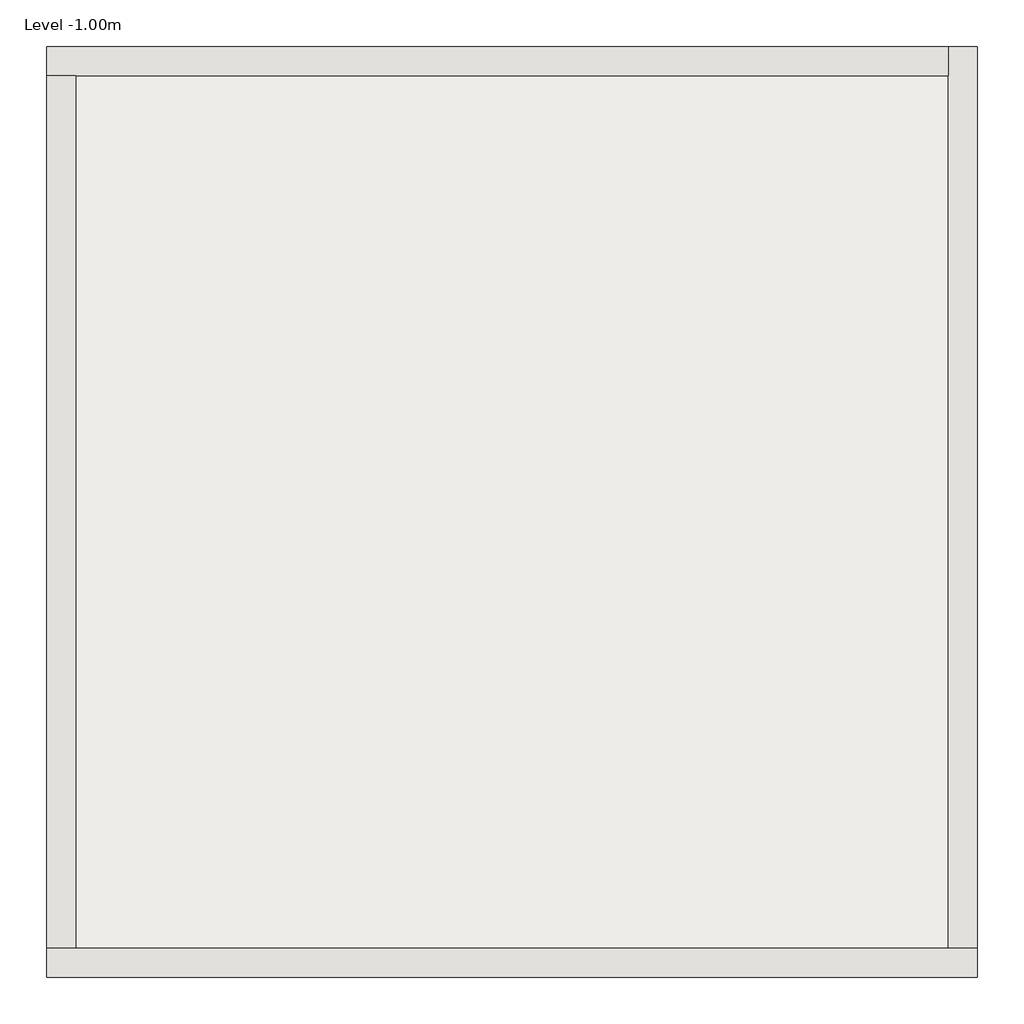
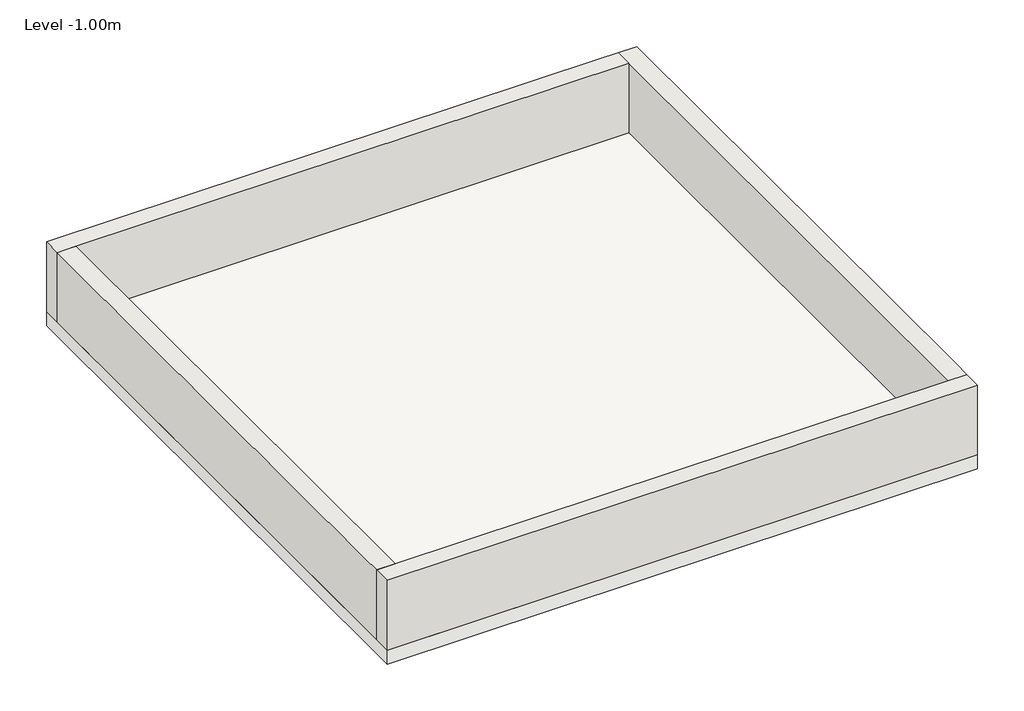
# One storey: 4 walls, 1 slab.
"""IFC4 building model written with IfcOpenShell, lengths in millimetres."""

from ifc_helpers import new_model, si_unit, frame, origin, place, context, project, spatial, polyline, outline, extrude, faceted_brep, element, save

model = new_model("IFC4")

# Units and contexts
model_context = context("Model", 3, world=origin())
ifc_project = project(units=[si_unit("LENGTHUNIT", "METRE", prefix="MILLI")], contexts=[model_context])

# Site, building, storey
site = spatial("IfcSite", under=ifc_project)
building = spatial("IfcBuilding", under=site)
storey = spatial("IfcBuildingStorey", under=building, Name="Level -1.00m", Elevation=-1000.0)

# Slab
placement = place(None, origin())
element("IfcSlab", 1, ObjectType="SOL CAM SANIT", at=placement, inside=storey, context=model_context, shape_type="SweptSolid", body=[
    extrude(outline(polyline([(0.0, 7999.99416), (7999.99416, 7999.99416), (7999.99416, 0.0), (0.0, 0.0), (0.0, 7999.99416)])), frame((0.0, 0.0, -1202.9999956), z_axis=(0.0, 0.0, 1.0), x_axis=(1.0, 0.0, 0.0)), (0.0, 0.0, 1.0), 202.9999956),
])

# Walls
element("IfcWall", 2, ObjectType="MURO CAM SANIT", at=placement, inside=storey, context=model_context, shape_type="Brep", body=[
    faceted_brep([(0.0, 0.0, -1000.0), (7999.99416, 0.0, -1000.0), (7999.99416, 0.0, -0.01216), (0.0, 0.0, -0.01216), (0.0, 249.000008, -1000.0), (0.0, 249.000008, -0.01216), (249.000008, 249.000008, -0.01216), (7750.994152, 249.000008, -0.01216), (7999.99416, 249.000008, -0.01216), (7999.99416, 249.000008, -1000.0), (7750.994152, 249.000008, -1000.0), (249.000008, 249.000008, -1000.0)], [[[0, 1, 2, 3]], [[4, 5, 6, 7, 8, 9, 10, 11]], [[1, 0, 4, 11, 10, 9]], [[3, 2, 8, 7, 6, 5]], [[2, 1, 9, 8]], [[0, 3, 5, 4]]]),
])
element("IfcWall", 3, ObjectType="MURO CAM SANIT", at=placement, inside=storey, context=model_context, shape_type="Brep", body=[
    faceted_brep([(7999.99416, 249.000008, -1000.0), (7999.99416, 7999.99416, -1000.0), (7999.99416, 7999.99416, -0.01216), (7999.99416, 500.000016, -0.01216), (7999.99416, 249.000008, -0.01216), (7750.994152, 249.000008, -1000.0), (7750.994152, 249.000008, -0.01216), (7750.994152, 7750.994152, -0.01216), (7750.994152, 7999.99416, -0.01216), (7750.994152, 7999.99416, -1000.0), (7750.994152, 7750.994152, -1000.0)], [[[0, 1, 2, 3, 4]], [[5, 6, 7, 8, 9, 10]], [[1, 0, 5, 10, 9]], [[4, 3, 2, 8, 7, 6]], [[2, 1, 9, 8]], [[0, 4, 6, 5]]]),
])
element("IfcWall", 4, ObjectType="MURO CAM SANIT", at=placement, inside=storey, context=model_context, shape_type="Brep", body=[
    faceted_brep([(7750.994152, 7999.99416, -1000.0), (0.0, 7999.99416, -1000.0), (0.0, 7999.99416, -0.01216), (7499.994144, 7999.99416, -0.01216), (7750.994152, 7999.99416, -0.01216), (7750.994152, 7750.994152, -1000.0), (7750.994152, 7750.994152, -0.01216), (249.000008, 7750.994152, -0.01216), (0.0, 7750.994152, -0.01216), (0.0, 7750.994152, -1000.0), (249.000008, 7750.994152, -1000.0)], [[[0, 1, 2, 3, 4]], [[5, 6, 7, 8, 9, 10]], [[1, 0, 5, 10, 9]], [[4, 3, 2, 8, 7, 6]], [[2, 1, 9, 8]], [[0, 4, 6, 5]]]),
])
element("IfcWall", 5, ObjectType="MURO CAM SANIT", at=placement, inside=storey, context=model_context, shape_type="Brep", body=[
    faceted_brep([(0.0, 7750.994152, -1000.0), (0.0, 249.000008, -1000.0), (0.0, 249.000008, -0.01216), (0.0, 500.000016, -0.01216), (0.0, 7499.994144, -0.01216), (0.0, 7750.994152, -0.01216), (249.000008, 7750.994152, -1000.0), (249.000008, 7750.994152, -0.01216), (249.000008, 249.000008, -0.01216), (249.000008, 249.000008, -1000.0)], [[[0, 1, 2, 3, 4, 5]], [[6, 7, 8, 9]], [[1, 0, 6, 9]], [[5, 4, 3, 2, 8, 7]], [[2, 1, 9, 8]], [[0, 5, 7, 6]]]),
])

save(model, "model.ifc")

# Revit data of these elements
# Project information
#   Organization Name = "Organization Name"
#   Organization Description = "Organization Description"
#   Building Name = "Building Name"
#   Project Issue Date = "Issue Date"
#   Project Status = "Project Status"
#   Client Name = "Client Name"
#   Project Address = "Enter address here\nAddress Line 2"
#   Project Name = "Project Name"
#   Project Number = "Project Number"
# Type "SOL CAM SANIT"
#   Layers, outside or top first: 0.080 m "Hormigón en masa d entre 2000 y 2300" (function 1); 0.003 m "Cloruro de polivinilo (PVC)" (function 1); 0.120 m "Arena y grava (d entre 1700 y 2200)" (function 1)
# Type "MURO CAM SANIT"
#   Description = "Metal Studs with Brick over sheathing on exterior and Gypsum Wall Board (GWB) on interior, Exterior Function"
#   Assembly Code = "B2010158"
#   Type Mark = "W10"
#   Layers, outside or top first: 0.009 m no material (function 1); 0.240 m no material (function 1)
# Element 1 (IfcSlab, "SOL CAM SANIT")
#   Height Offset From Level = 0.000 m
#   Phase Created = New Construction
#   Materials on its faces: "Arena y grava (d entre 1700 y 2200)", "Hormigón en masa d entre 2000 y 2300"
# Elements 2, 3, 4, 5 (IfcWall, "MURO CAM SANIT")
#   Comments = "BEM_GROUND_COUPLED"
#   Top Offset = 0.000 m
#   Base Offset = 0.000 m
#   Unconnected Height = 0.999988 m
#   wall height = 0.999988 m
#   Phase Created = New Construction
#   Base Constraint = Level -1.00m
#   Materials on its faces: "Default Wall"
# Materials
#   "Hormigón en masa d entre 2000 y 2300": class "Unassigned", colour RGB 0 0 0, transparency 0
#   "Cloruro de polivinilo (PVC)": class "Unassigned", colour RGB 0 0 0, transparency 0
#   "Arena y grava (d entre 1700 y 2200)": class "Unassigned", colour RGB 0 0 0, transparency 0
#   "Default Wall": class "Miscellaneous", colour RGB 192 192 192, transparency 0, Cost = 0
